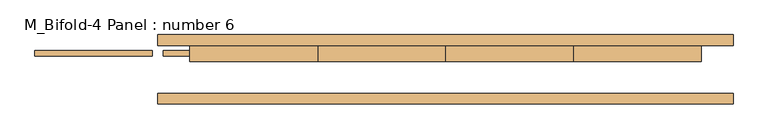
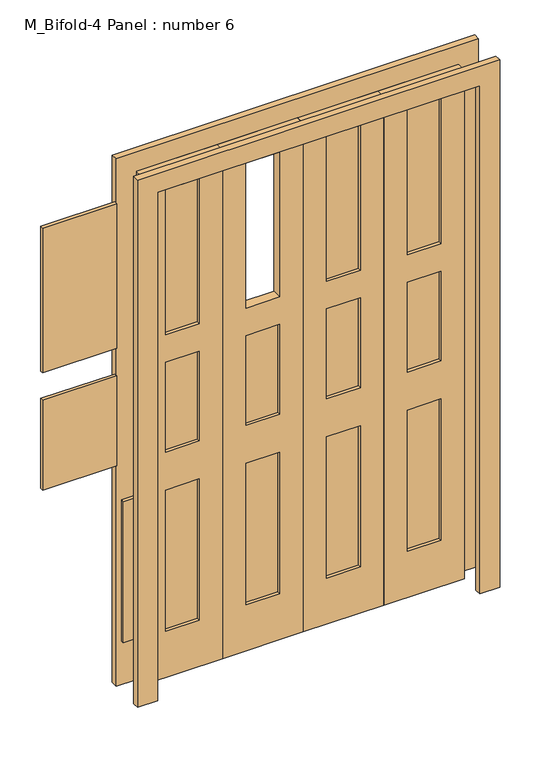
"""IFC4 building model written with IfcOpenShell, lengths in millimetres: door geometry, M_Bifold-4 Panel : number 6."""

from ifc_helpers import new_model, si_unit, frame, origin, place, context, project, spatial, polyline, outline, extrude, source, transform, mapped, element, save


def m_bifold_4_panel_number_6_3b3d9f7e(model_context):
    return source(origin(), model_context, "Body", "SweptSolid", [
        extrude(outline(polyline([(393.7, 44.45), (520.7, 44.45), (520.7, 31.75), (393.7, 31.75), (393.7, 44.45)])), frame((0.0, 0.0, 1370.1314325), z_axis=(0.0, 0.0, 1.0), x_axis=(1.0, 0.0, 0.0)), (0.0, 0.0, 1.0), 579.3185675),
        extrude(outline(polyline([(393.7, 44.45), (520.7, 44.45), (520.7, 31.75), (393.7, 31.75), (393.7, 44.45)])), frame((0.0, 0.0, 184.15), z_axis=(0.0, 0.0, 1.0), x_axis=(1.0, 0.0, 0.0)), (0.0, 0.0, 1.0), 565.15),
        extrude(outline(polyline([(-63.8, 44.45), (215.9, 44.45), (215.9, 31.75), (-63.8, 31.75), (-63.8, 44.45)])), frame((0.0, 0.0, 1370.1314325), z_axis=(0.0, 0.0, 1.0), x_axis=(1.0, 0.0, 0.0)), (0.0, 0.0, 1.0), 579.3185675),
        extrude(outline(polyline([(88.9, 44.45), (215.9, 44.45), (215.9, 31.75), (88.9, 31.75), (88.9, 44.45)])), frame((0.0, 0.0, 184.15), z_axis=(0.0, 0.0, 1.0), x_axis=(1.0, 0.0, 0.0)), (0.0, 0.0, 1.0), 565.15),
        extrude(outline(polyline([(-215.9, 44.45), (-88.9, 44.45), (-88.9, 31.75), (-215.9, 31.75), (-215.9, 44.45)])), frame((0.0, 0.0, 184.15), z_axis=(0.0, 0.0, 1.0), x_axis=(1.0, 0.0, 0.0)), (0.0, 0.0, 1.0), 565.15),
        extrude(outline(polyline([(-521.3, 44.45), (-241.6, 44.45), (-241.6, 31.75), (-521.3, 31.75), (-521.3, 44.45)])), frame((0.0, 0.0, 1370.1314325), z_axis=(0.0, 0.0, 1.0), x_axis=(1.0, 0.0, 0.0)), (0.0, 0.0, 1.0), 579.3185675),
        extrude(outline(polyline([(-978.8, 44.45), (-699.1, 44.45), (-699.1, 31.75), (-978.8, 31.75), (-978.8, 44.45)])), frame((0.0, 0.0, 1370.1314325), z_axis=(0.0, 0.0, 1.0), x_axis=(1.0, 0.0, 0.0)), (0.0, 0.0, 1.0), 579.3185675),
        extrude(outline(polyline([(-673.4, 44.45), (-393.7, 44.45), (-393.7, 31.75), (-673.4, 31.75), (-673.4, 44.45)])), frame((0.0, 0.0, 184.15), z_axis=(0.0, 0.0, 1.0), x_axis=(1.0, 0.0, 0.0)), (0.0, 0.0, 1.0), 565.15),
        extrude(outline(polyline([(-521.3, 44.45), (-88.9, 44.45), (-88.9, 31.75), (-521.3, 31.75), (-521.3, 44.45)])), frame((0.0, 0.0, 901.1314325), z_axis=(0.0, 0.0, 1.0), x_axis=(1.0, 0.0, 0.0)), (0.0, 0.0, 1.0), 359.3185675),
        extrude(outline(polyline([(88.9, 44.45), (215.9, 44.45), (215.9, 31.75), (88.9, 31.75), (88.9, 44.45)])), frame((0.0, 0.0, 901.1314325), z_axis=(0.0, 0.0, 1.0), x_axis=(1.0, 0.0, 0.0)), (0.0, 0.0, 1.0), 359.3185675),
        extrude(outline(polyline([(393.7, 44.45), (520.7, 44.45), (520.7, 31.75), (393.7, 31.75), (393.7, 44.45)])), frame((0.0, 0.0, 901.1314325), z_axis=(0.0, 0.0, 1.0), x_axis=(1.0, 0.0, 0.0)), (0.0, 0.0, 1.0), 359.3185675),
        extrude(outline(polyline([(-978.8, 44.45), (-699.1, 44.45), (-699.1, 31.75), (-978.8, 31.75), (-978.8, 44.45)])), frame((0.0, 0.0, 901.1314325), z_axis=(0.0, 0.0, 1.0), x_axis=(1.0, 0.0, 0.0)), (0.0, 0.0, 1.0), 359.3185675),
        extrude(outline(polyline([(0.0, 685.6), (2108.0, 685.6), (2108.0, -685.6), (0.0, -685.6), (0.0, -609.6), (2032.0, -609.6), (2032.0, 609.6), (0.0, 609.6), (0.0, 685.6)])), frame((0.0, -82.55, 0.0), z_axis=(0.0, 1.0, 0.0), x_axis=(0.0, 0.0, 1.0)), (0.0, 0.0, 1.0), 25.4),
        extrude(outline(polyline([(0.0, 685.6), (2108.0, 685.6), (2108.0, -685.6), (0.0, -685.6), (0.0, -609.6), (2032.0, -609.6), (2032.0, 609.6), (0.0, 609.6), (0.0, 685.6)])), frame((0.0, 57.15, 0.0), z_axis=(0.0, 1.0, 0.0), x_axis=(0.0, 0.0, 1.0)), (0.0, 0.0, 1.0), 25.4),
        extrude(outline(polyline([(0.0, -609.6), (0.0, -304.8), (2032.0, -304.8), (2032.0, -609.6), (0.0, -609.6)]), holes=[polyline([(1949.45, -520.7), (1949.45, -393.7), (1370.1314325, -393.7), (1370.1314325, -520.7), (1949.45, -520.7)]), polyline([(749.3, -520.7), (749.3, -393.7), (184.15, -393.7), (184.15, -520.7), (749.3, -520.7)]), polyline([(1260.45, -520.7), (1260.45, -393.7), (901.1314325, -393.7), (901.1314325, -520.7), (1260.45, -520.7)])]), frame((0.0, 19.05, 0.0), z_axis=(0.0, 1.0, 0.0), x_axis=(0.0, 0.0, 1.0)), (0.0, 0.0, 1.0), 38.1),
        extrude(outline(polyline([(0.0, -304.8), (0.0, 0.0), (2032.0, 0.0), (2032.0, -304.8), (0.0, -304.8)]), holes=[polyline([(1949.45, -215.9), (1949.45, -88.9), (1370.1314325, -88.9), (1370.1314325, -215.9), (1949.45, -215.9)]), polyline([(749.3, -215.9), (749.3, -88.9), (184.15, -88.9), (184.15, -215.9), (749.3, -215.9)]), polyline([(1260.45, -215.9), (1260.45, -88.9), (901.1314325, -88.9), (901.1314325, -215.9), (1260.45, -215.9)])]), frame((0.0, 19.05, 0.0), z_axis=(0.0, 1.0, 0.0), x_axis=(0.0, 0.0, 1.0)), (0.0, 0.0, 1.0), 38.1),
        extrude(outline(polyline([(0.0, 0.0), (0.0, 304.8), (2032.0, 304.8), (2032.0, 0.0), (0.0, 0.0)]), holes=[polyline([(1949.45, 88.9), (1949.45, 215.9), (1370.1314325, 215.9), (1370.1314325, 88.9), (1949.45, 88.9)]), polyline([(749.3, 88.9), (749.3, 215.9), (184.15, 215.9), (184.15, 88.9), (749.3, 88.9)]), polyline([(1260.45, 88.9), (1260.45, 215.9), (901.1314325, 215.9), (901.1314325, 88.9), (1260.45, 88.9)])]), frame((0.0, 19.05, 0.0), z_axis=(0.0, 1.0, 0.0), x_axis=(0.0, 0.0, 1.0)), (0.0, 0.0, 1.0), 38.1),
        extrude(outline(polyline([(0.0, 304.8), (0.0, 609.6), (2032.0, 609.6), (2032.0, 304.8), (0.0, 304.8)]), holes=[polyline([(1949.45, 393.7), (1949.45, 520.7), (1370.1314325, 520.7), (1370.1314325, 393.7), (1949.45, 393.7)]), polyline([(749.3, 393.7), (749.3, 520.7), (184.15, 520.7), (184.15, 393.7), (749.3, 393.7)]), polyline([(1260.45, 393.7), (1260.45, 520.7), (901.1314325, 520.7), (901.1314325, 393.7), (1260.45, 393.7)])]), frame((0.0, 19.05, 0.0), z_axis=(0.0, 1.0, 0.0), x_axis=(0.0, 0.0, 1.0)), (0.0, 0.0, 1.0), 38.1),
    ])


if __name__ == "__main__":
    model = new_model("IFC4")
    model_context = context("Model", 3, world=origin())
    ifc_project = project(units=[si_unit("LENGTHUNIT", "METRE", prefix="MILLI")], contexts=[model_context])
    site = spatial("IfcSite", under=ifc_project)
    building = spatial("IfcBuilding", under=site)
    placement = place(None, origin())
    m_bifold_4_panel_number_6_shape = m_bifold_4_panel_number_6_3b3d9f7e(model_context)
    element("IfcDoor", 1, ObjectType="M_Bifold-4 Panel : number 6", at=placement, inside=building, context=model_context, shape_type="MappedRepresentation", body=[
        mapped(m_bifold_4_panel_number_6_shape, transform((0.0, 0.0, 0.0), x_axis=(1.0, 0.0, 0.0), y_axis=(0.0, 1.0, 0.0), z_axis=(0.0, 0.0, 1.0))),
    ])
    save(model, "model.ifc")

# Revit data of these elements
# Type "M_Bifold-4 Panel : number 6"
#   Type Mark = "93"
#   Analytic Construction = "<None>"
#   Thickness = 0' - 1 3/4"
#   Height = 6' - 8"
#   Trim Width = 0' - 2.99213"
#   Width = 4' - 0"
#   Define Thermal Properties by = 1
#   Door Material = Door - Panel
#   Frame Material = Door - Frame
#   Function = (empty or 0)
#   Assembly Code = ""
#   Description = (empty or 0)
#   Wall Closure = (empty or 0)
# Element 1 (IfcDoor, "M_Bifold-4 Panel : number 6")
#   Materials on its faces: "Door - Panel", "Door - Frame"
# Materials
#   "Door - Panel": class "Wood", colour RGB 210 159 95, transparency 0, Keynote = "L20", Cost = 0
#   "Door - Frame": class "Miscellaneous", colour RGB 118 70 51, transparency 0
